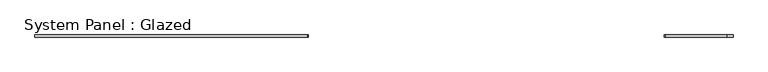
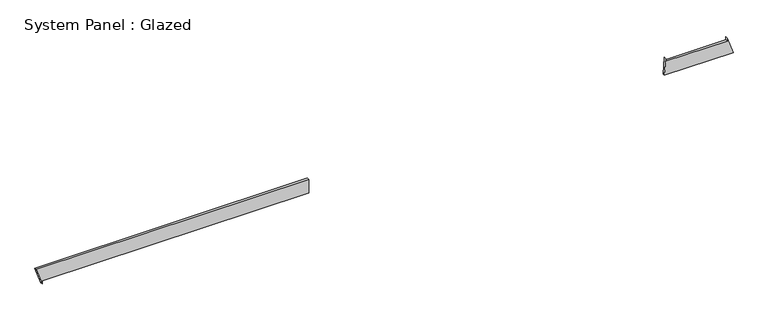
"""IFC4 building model written with IfcOpenShell, lengths in millimetres: plate geometry, System Panel : Glazed."""

import ifcopenshell
import ifcopenshell.guid

model = None  # the IFC model being written
_history = None  # IfcOwnerHistory: only IFC2X3 demands one
_inside = {}  # id of a spatial element -> (the spatial element, [elements in it])
_under = {}  # id of a project, library or spatial element -> (it, [spatial elements below it])
_declared = {}  # id of a project -> (the project, [libraries it declares])
_typed = {}  # id of a type object -> (the type object, [elements of that type])
_made_of = {}  # id of a material, layer set ... -> (it, [elements and type objects made of it])


def new_model(schema):
    """Start an empty IFC model of exactly this schema.

    Asked for "IFC4X3", IfcOpenShell would pick the latest addendum, in which some entities
    have other attributes; the version numbers below select the first issue.
    IFC2X3 requires an IfcOwnerHistory on every rooted entity: one is made here for all.
    """
    global model, _history
    if schema == "IFC4X3":
        model = ifcopenshell.file(schema_version=(4, 3, 0, 0))
    else:
        model = ifcopenshell.file(schema=schema)
    _inside.clear()
    _under.clear()
    _declared.clear()
    _typed.clear()
    _made_of.clear()
    _history = None
    if model.schema == "IFC2X3":
        org = make("IfcOrganization", Name="unknown")
        user = make(
            "IfcPersonAndOrganization",
            ThePerson=make("IfcPerson", FamilyName="unknown"),
            TheOrganization=org,
        )
        app = make(
            "IfcApplication",
            ApplicationDeveloper=org,
            Version="unknown",
            ApplicationFullName="unknown",
            ApplicationIdentifier="unknown",
        )
        _history = make(
            "IfcOwnerHistory",
            OwningUser=user,
            OwningApplication=app,
            ChangeAction="ADDED",
            CreationDate=0,
        )
    return model


def make(cls, **values):
    """One entity of the class cls with the attributes given. An attribute that is None is left unset."""
    return model.create_entity(
        cls, **{name: value for name, value in values.items() if value is not None}
    )


def rooted(cls, **values):
    """An entity with a GlobalId (a new one), such as an element, a storey or a relation."""
    return make(cls, GlobalId=ifcopenshell.guid.new(), OwnerHistory=_history, **values)


def si_unit(unit_type, name, prefix=None):
    """IfcSIUnit, for example si_unit("LENGTHUNIT", "METRE", prefix="MILLI")."""
    return make("IfcSIUnit", UnitType=unit_type, Prefix=prefix, Name=name)


def assignment(units):
    """IfcUnitAssignment: the units of a project."""
    return None if units is None else make("IfcUnitAssignment", Units=units)


def point(xyz):
    """IfcCartesianPoint."""
    return None if xyz is None else make("IfcCartesianPoint", Coordinates=xyz)


def direction(xyz):
    """IfcDirection."""
    return None if xyz is None else make("IfcDirection", DirectionRatios=xyz)


def frame(location, z_axis=None, x_axis=None):
    """IfcAxis2Placement3D, a coordinate frame: its origin and axes. An axis left out is left unset."""
    return make(
        "IfcAxis2Placement3D",
        Location=point(location),
        Axis=direction(z_axis),
        RefDirection=direction(x_axis),
    )


def origin():
    """The frame at (0, 0, 0) with its axes left unset."""
    return frame((0.0, 0.0, 0.0))


def place(relative_to, where):
    """IfcLocalPlacement: puts the frame where relative to a parent placement (None: the world)."""
    return make(
        "IfcLocalPlacement", PlacementRelTo=relative_to, RelativePlacement=where
    )


def context(
    kind, dimensions, precision=None, world=None, true_north=None, identifier=None
):
    """IfcGeometricRepresentationContext, for example the 3D "Model" context."""
    return make(
        "IfcGeometricRepresentationContext",
        ContextIdentifier=identifier,
        ContextType=kind,
        CoordinateSpaceDimension=dimensions,
        Precision=precision,
        WorldCoordinateSystem=world,
        TrueNorth=true_north,
    )


def project(units=None, contexts=None):
    """IfcProject with its units and contexts."""
    return rooted(
        "IfcProject",
        Name="project",
        RepresentationContexts=contexts,
        UnitsInContext=assignment(units),
    )


def spatial(cls, under=None, at=None, **own):
    """A site, building, storey or space (cls), placed at a placement, below another one or the project."""
    s = rooted(cls, ObjectPlacement=at, **own)
    if under is not None:
        _under.setdefault(under.id(), (under, []))[1].append(s)
    return s


def polyline(points):
    """IfcPolyline through the points."""
    return make("IfcPolyline", Points=[point(p) for p in points])


def outline(outer, holes=None, kind="AREA"):
    """IfcArbitraryClosedProfileDef: a profile drawn as a closed curve; with holes, ...WithVoids."""
    if holes is None:
        return make("IfcArbitraryClosedProfileDef", ProfileType=kind, OuterCurve=outer)
    return make(
        "IfcArbitraryProfileDefWithVoids",
        ProfileType=kind,
        OuterCurve=outer,
        InnerCurves=holes,
    )


def extrude(swept, where, along, depth):
    """IfcExtrudedAreaSolid: the profile swept, set in the frame where, extruded along a direction by depth."""
    return make(
        "IfcExtrudedAreaSolid",
        SweptArea=swept,
        Position=where,
        ExtrudedDirection=direction(along),
        Depth=depth,
    )


def shape(context_of_items, identifier, shape_type, items):
    """IfcShapeRepresentation: the items that make up one representation, for example the "Body"."""
    return make(
        "IfcShapeRepresentation",
        ContextOfItems=context_of_items,
        RepresentationIdentifier=identifier,
        RepresentationType=shape_type,
        Items=items,
    )


def source(mapping_origin, context_of_items, identifier, shape_type, items):
    """IfcRepresentationMap: a shape defined once, which mapped items show again and again."""
    return make(
        "IfcRepresentationMap",
        MappingOrigin=mapping_origin,
        MappedRepresentation=shape(context_of_items, identifier, shape_type, items),
    )


def transform(
    local_origin,
    x_axis=None,
    y_axis=None,
    z_axis=None,
    scale=None,
    scale2=None,
    scale3=None,
    uniform=True,
):
    """IfcCartesianTransformationOperator3D, or its non-uniform kind. x_axis, y_axis, z_axis: its Axis1, 2, 3."""
    if uniform:
        return make(
            "IfcCartesianTransformationOperator3D",
            Axis1=direction(x_axis),
            Axis2=direction(y_axis),
            LocalOrigin=point(local_origin),
            Scale=scale,
            Axis3=direction(z_axis),
        )
    return make(
        "IfcCartesianTransformationOperator3DnonUniform",
        Axis1=direction(x_axis),
        Axis2=direction(y_axis),
        LocalOrigin=point(local_origin),
        Scale=scale,
        Axis3=direction(z_axis),
        Scale2=scale2,
        Scale3=scale3,
    )


def mapped(mapping_source, mapping_target):
    """IfcMappedItem: shows the shape of a source again, moved by a transform."""
    return make(
        "IfcMappedItem", MappingSource=mapping_source, MappingTarget=mapping_target
    )


def made_of(thing, what):
    """Note that an element or type object is made of a material, layer set ...; save() writes the relation."""
    if what is not None:
        _made_of.setdefault(what.id(), (what, []))[1].append(thing)
    return thing


def element(
    cls,
    number,
    at=None,
    inside=None,
    cuts=None,
    type_object=None,
    material=None,
    context=None,
    identifier="Body",
    shape_type=None,
    held_by="IfcProductDefinitionShape",
    body=None,
    shapes=None,
    **own,
):
    """One element of the class cls, such as IfcWall. Its Tag is "e" and its number.

    at: its placement. inside: the storey or other place that contains it. cuts: it is an
    opening in that element (IfcRelVoidsElement). A single representation is given by context,
    identifier, shape_type and body (its items); several are given by shapes. held_by: the class
    of the entity that holds the representations. save() writes the other relations.
    """
    e = rooted(cls, Tag="e%d" % number, ObjectPlacement=at, **own)
    if body is not None:
        shapes = [shape(context, identifier, shape_type, body)]
    if shapes is not None:
        e.Representation = make(held_by, Representations=shapes)
    if inside is not None:
        _inside.setdefault(inside.id(), (inside, []))[1].append(e)
    if cuts is not None:
        rooted(
            "IfcRelVoidsElement", RelatingBuildingElement=cuts, RelatedOpeningElement=e
        )
    if type_object is not None:
        _typed.setdefault(type_object.id(), (type_object, []))[1].append(e)
    return made_of(e, material)


def aggregate(whole, parts):
    """IfcRelAggregates: a whole, such as a stair, and the parts it consists of."""
    return rooted("IfcRelAggregates", RelatingObject=whole, RelatedObjects=parts)


def save(model, path):
    """Write the relations noted so far, then the file.

    IfcRelAggregates (storeys below a building ...), IfcRelContainedInSpatialStructure (elements
    in a storey), IfcRelDefinesByType, IfcRelAssociatesMaterial and IfcRelDeclares: one each for
    every whole, place, type object, material and project.
    """
    for whole, parts in _under.values():
        aggregate(whole, parts)
    for where, things in _inside.values():
        rooted(
            "IfcRelContainedInSpatialStructure",
            RelatedElements=things,
            RelatingStructure=where,
        )
    for kind, things in _typed.values():
        rooted("IfcRelDefinesByType", RelatedObjects=things, RelatingType=kind)
    for what, things in _made_of.values():
        rooted("IfcRelAssociatesMaterial", RelatedObjects=things, RelatingMaterial=what)
    for by, libraries in _declared.values():
        rooted("IfcRelDeclares", RelatingContext=by, RelatedDefinitions=libraries)
    model.write(path)


def system_panel_glazed_dba537f6(model_context):
    return source(origin(), model_context, "Body", "SweptSolid", [
        extrude(outline(polyline([(35.3553391, 3233.2334966), (35.3553391, 4027.7930193), (235.7005018, 3958.9828813), (200.3451627, 3958.98343), (200.3341084, 3246.7911885), (235.6894474, 3246.7906397), (35.3553391, 3233.2334966)])), frame((0.0, -49.5, 0.0), z_axis=(0.0, 1.0, 0.0), x_axis=(0.0, 0.0, 1.0)), (0.0, 0.0, 1.0), 25.0),
        extrude(outline(polyline([(0.0, -3958.6827411), (35.3553391, -3958.6827411), (35.3553391, -875.2968038), (200.2700807, -878.2816654), (200.2211953, -4027.7930193), (0.0, -3958.6827411)])), frame((0.0, -49.5, 0.0), z_axis=(0.0, 1.0, 0.0), x_axis=(0.0, 0.0, 1.0)), (0.0, 0.0, 1.0), 25.0),
    ])


if __name__ == "__main__":
    model = new_model("IFC4")
    model_context = context("Model", 3, world=origin())
    ifc_project = project(units=[si_unit("LENGTHUNIT", "METRE", prefix="MILLI")], contexts=[model_context])
    site = spatial("IfcSite", under=ifc_project)
    building = spatial("IfcBuilding", under=site)
    placement = place(None, origin())
    system_panel_glazed_shape = system_panel_glazed_dba537f6(model_context)
    element("IfcPlate", 1, ObjectType="System Panel : Glazed", at=placement, inside=building, context=model_context, shape_type="MappedRepresentation", body=[
        mapped(system_panel_glazed_shape, transform((0.0, 0.0, 0.0), x_axis=(1.0, 0.0, 0.0), y_axis=(0.0, 1.0, 0.0), z_axis=(0.0, 0.0, 1.0))),
    ])
    save(model, "model.ifc")

# Revit data of these elements
# Element 1 (IfcPlate, "System Panel : Glazed")
#   Materials on its faces: "Glass"
# Materials
#   "Glass": class "Glass", colour RGB 218 227 224, transparency 0.85, Description = "Soda Lime Glass", Cost = 0
